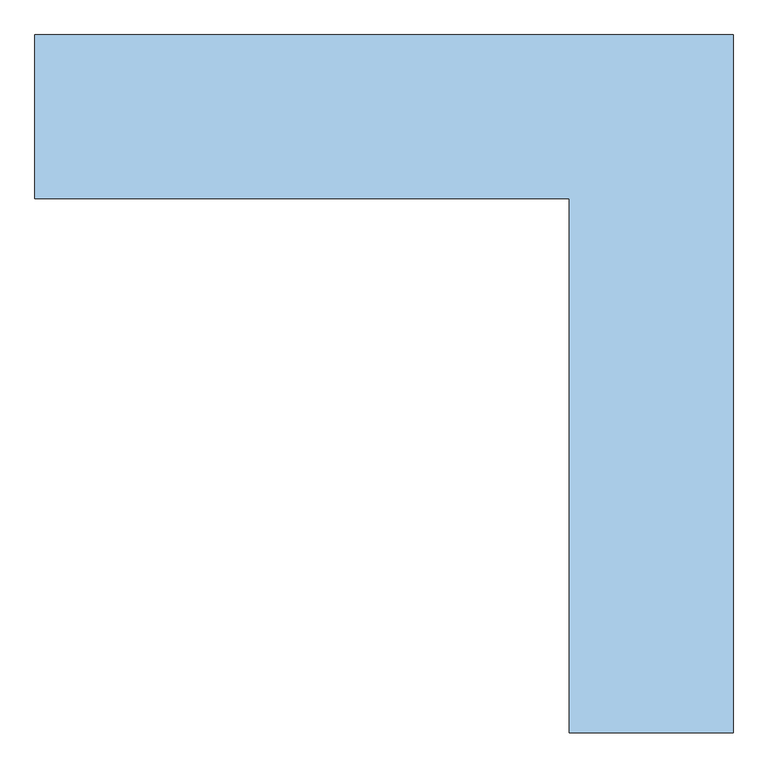
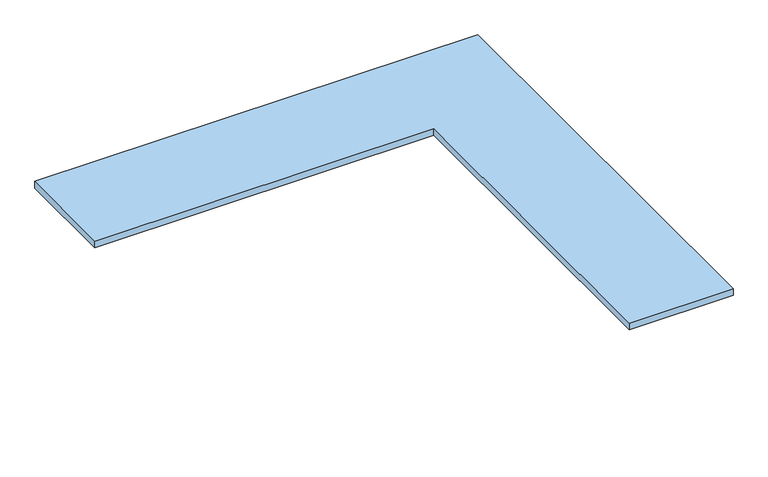
"""IFC4 building model written with IfcOpenShell, lengths in millimetres: window geometry, .CC_ND 300_PEDRA PEITORIL EM L : 1.26F x 1.26E x 0.30L."""

from ifc_helpers import new_model, si_unit, frame, origin, place, context, project, spatial, polyline, outline, extrude, source, transform, mapped, element, save


def window_94eaf2cf(model_context):
    return source(origin(), model_context, "Body", "SweptSolid", [
        extrude(outline(polyline([(-615.0, -147.5), (-615.0, 148.0), (645.0, 148.0), (645.0, -1112.0), (349.5, -1112.0), (349.5, -147.5), (-615.0, -147.5)])), frame((0.0, 0.0, 900.0), z_axis=(0.0, 0.0, 1.0), x_axis=(1.0, 0.0, 0.0)), (0.0, 0.0, 1.0), 20.0),
    ])


if __name__ == "__main__":
    model = new_model("IFC4")
    model_context = context("Model", 3, world=origin())
    ifc_project = project(units=[si_unit("LENGTHUNIT", "METRE", prefix="MILLI")], contexts=[model_context])
    site = spatial("IfcSite", under=ifc_project)
    building = spatial("IfcBuilding", under=site)
    placement = place(None, origin())
    window_shape = window_94eaf2cf(model_context)
    element("IfcWindow", 1, ObjectType=".CC_ND 300_PEDRA PEITORIL EM L : 1.26F x 1.26E x 0.30L", at=placement, inside=building, context=model_context, shape_type="MappedRepresentation", body=[
        mapped(window_shape, transform((0.0, 0.0, 0.0), x_axis=(1.0, 0.0, 0.0), y_axis=(0.0, 1.0, 0.0), z_axis=(0.0, 0.0, 1.0))),
    ])
    save(model, "model.ifc")

# Revit data of these elements
# Type ".CC_ND 300_PEDRA PEITORIL EM L : 1.26F x 1.26E x 0.30L"
#   Type Mark = "73"
#   Largura da pedra da frente [instance default] = 0.26 m
#   Largura da pedra da esquerda [instance default] = 0.26 m
#   Extensão esquerda interna [instance default] = 0.03 m
#   Extensão esquerda externa [instance default] = 0.03 m
#   Comprimento Esquerda = 0.9645 m
#   Extensão frente interna [instance default] = 0.03 m
#   Extensão frente externa [instance default] = 0.03 m
#   Espessura peitoril = 0.02 m
#   Espessura da parede [instance default] = 0.20 m
#   Comprimento da pedra [instance default] = 2.1945 m
#   Comprimento Frente = 1.23 m
#   Altura-padrão do peitoril [instance default] = 0.90 m
#   Pedra do peitoril = .GRANITO_BRANCO_ITAUNAS
#   Rough Width = 0
#   Rough Height = 0
#   Height = 0
#   Wall Closure = (empty or 0)
#   Width = 0
# Element 1 (IfcWindow, ".CC_ND 300_PEDRA PEITORIL EM L : 1.26F x 1.26E x 0.30L")
#   Largura da pedra da frente = 0.2955 m
#   Largura da pedra da esquerda = 0.2955 m
#   Extensão esquerda interna = 0.0295 m
#   Extensão frente interna = 0.0295 m
#   Espessura da parede = 0.236 m
#   Materials on its faces: ".GRANITO_BRANCO_ITAUNAS"
# Materials
#   ".GRANITO_BRANCO_ITAUNAS": class ".CC_PEDRA REVEST.", colour RGB 202 195 174, transparency 0, Description = "Revestimento em granito", Cost = 0
